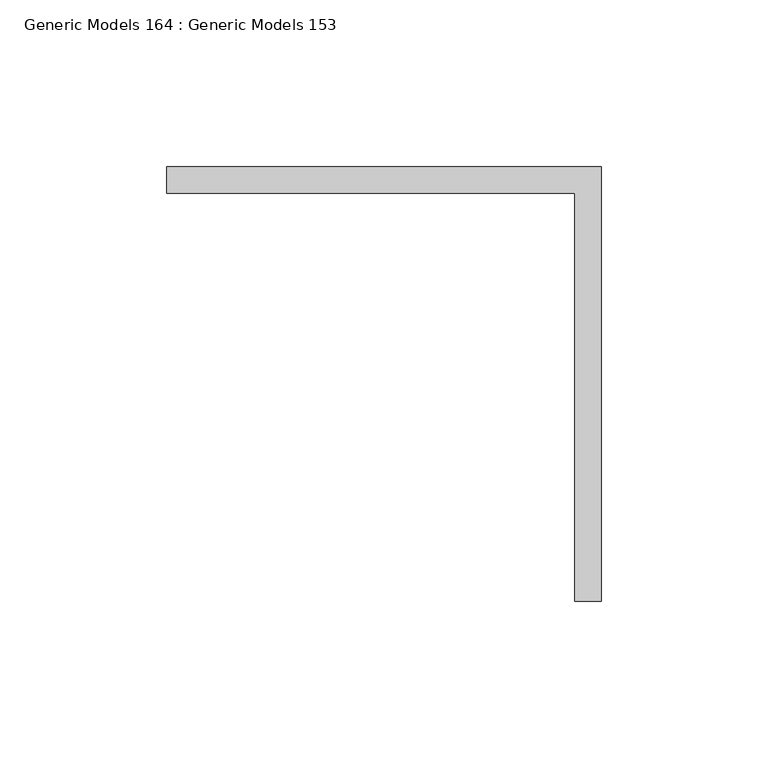
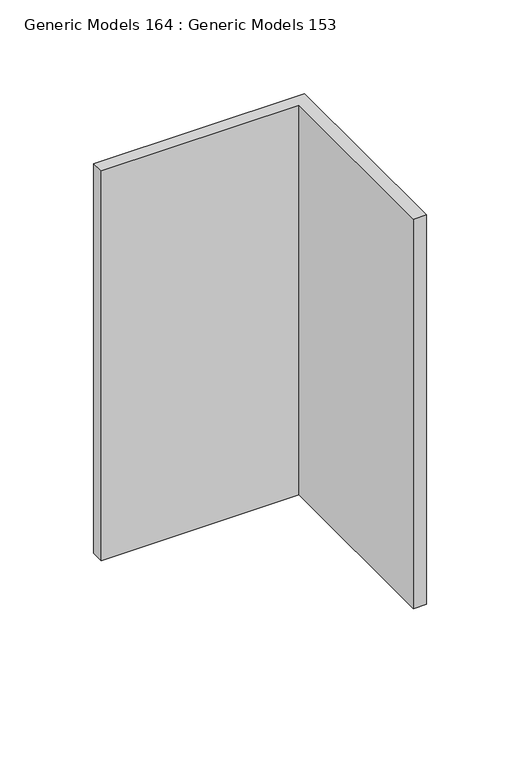
"""IFC4 building model written with IfcOpenShell, lengths in millimetres: proxy geometry, Generic Models 164 : Generic Models 153."""

from ifc_helpers import new_model, si_unit, frame, origin, place, context, project, spatial, polyline, outline, extrude, source, transform, mapped, element, save


def generic_models_164_generic_models_153_ac50f4f0(model_context):
    return source(origin(), model_context, "Body", "SweptSolid", [
        extrude(outline(polyline([(31762.6846032, 36207.3957942), (31762.6846032, 36329.6332942), (31640.4471032, 36329.6332942), (31640.4471032, 36337.5707942), (31770.6221032, 36337.5707942), (31770.6221032, 36207.3957942), (31762.6846032, 36207.3957942)])), frame((0.0, 0.0, 271626.0125), z_axis=(0.0, 0.0, 1.0), x_axis=(1.0, 0.0, 0.0)), (0.0, 0.0, 1.0), 254.0),
    ])


if __name__ == "__main__":
    model = new_model("IFC4")
    model_context = context("Model", 3, world=origin())
    ifc_project = project(units=[si_unit("LENGTHUNIT", "METRE", prefix="MILLI")], contexts=[model_context])
    site = spatial("IfcSite", under=ifc_project)
    building = spatial("IfcBuilding", under=site)
    placement = place(None, origin())
    generic_models_164_generic_models_153_shape = generic_models_164_generic_models_153_ac50f4f0(model_context)
    element("IfcBuildingElementProxy", 1, Name="Generic Models 164 : Generic Models 153", ObjectType="Generic Models 164 : Generic Models 153", at=placement, inside=building, context=model_context, shape_type="MappedRepresentation", body=[
        mapped(generic_models_164_generic_models_153_shape, transform((0.0, 0.0, 0.0), x_axis=(1.0, 0.0, 0.0), y_axis=(0.0, 1.0, 0.0), z_axis=(0.0, 0.0, 1.0))),
    ])
    save(model, "model.ifc")
